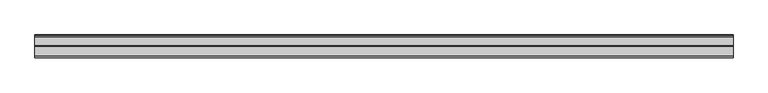
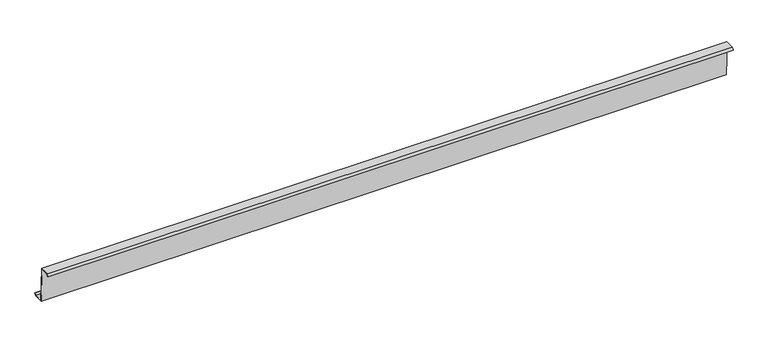
"""IFC4 building model written with IfcOpenShell, lengths in millimetres: proxy geometry, Generic Models 7:Generic Models 1:8:Generic Models 1:8 : Generic Models 7:Generic Models 1:337419:32 : Generic Models 7:Generic Models 1:8:Generic Models 1:8 : Generic Models 7:Generic Models 1:337419:315935."""

from ifc_helpers import new_model, si_unit, frame, origin, place, context, project, spatial, polyline, outline, extrude, source, transform, mapped, element, save


def generic_models_b363cb20(model_context):
    return source(origin(), model_context, "Body", "SweptSolid", [
        extrude(outline(polyline([(-574595.2827823, 4107.9663588), (-574530.4499739, 4110.6677258), (-574519.9914704, 3859.6636418), (-574459.2287164, 3862.1954233), (-574448.3924197, 3876.2595027), (-574446.191756, 3874.5639032), (-574457.8187237, 3859.4736374), (-574522.6515321, 3856.7722704), (-574533.1100356, 4107.7763544), (-574593.8424733, 4105.2458362), (-574604.690674, 4091.166307), (-574606.90975, 4092.876093), (-574595.2827823, 4107.9663588)])), frame((591306.0367239, 0.0, 0.0), z_axis=(1.0, 0.0, 0.0), x_axis=(0.0, 1.0, 0.0)), (0.0, 0.0, 1.0), 4876.8),
    ])


if __name__ == "__main__":
    model = new_model("IFC4")
    model_context = context("Model", 3, world=origin())
    ifc_project = project(units=[si_unit("LENGTHUNIT", "METRE", prefix="MILLI")], contexts=[model_context])
    site = spatial("IfcSite", under=ifc_project)
    building = spatial("IfcBuilding", under=site)
    placement = place(None, origin())
    generic_models_shape = generic_models_b363cb20(model_context)
    element("IfcBuildingElementProxy", 1, Name="Generic Models 7:Generic Models 1:8:Generic Models 1:8 : Generic Models 7:Generic Models 1:337419:32 : Generic Models 7:Generic Models 1:8:Generic Models 1:8 : Generic Models 7:Generic Models 1:337419:315935", ObjectType="Generic Models 7:Generic Models 1:8:Generic Models 1:8 : Generic Models 7:Generic Models 1:337419:32 : Generic Models 7:Generic Models 1:8:Generic Models 1:8 : Generic Models 7:Generic Models 1:337419:315935", at=placement, inside=building, context=model_context, shape_type="MappedRepresentation", body=[
        mapped(generic_models_shape, transform((0.0, 0.0, 0.0), x_axis=(1.0, 0.0, 0.0), y_axis=(0.0, 1.0, 0.0), z_axis=(0.0, 0.0, 1.0))),
    ])
    save(model, "model.ifc")

# Revit data of these elements
# Type "Generic Models 7:Generic Models 1:8:Generic Models 1:8 : Generic Models 7:Generic Models 1:337419:32 : Generic Models 7:Generic Models 1:8:Generic Models 1:8 : Generic Models 7:Generic Models 1:337419:315935"
#   NameOverride = "Generic Models 7:Generic Models 1:8:Generic Models 1:8 : Generic Models 7:Generic Models 1:337419:315935"
#   ObjectTypeOverride = "Generic Models 1:8 : Generic Models 7:Generic Models 1:337419"
#   Reference = "Generic Models 1"
#   Tag = "315935"
# Element 1 (IfcBuildingElementProxy, "Generic Models 7:Generic Models 1:8:Generic Models 1:8 : Generic Models 7:Generic Models 1:337419:32 : Generic Models 7:Generic Models 1:8:Generic Models 1:8 : Generic Models 7:Generic Models 1:337419:315935")
#   Materials on its faces: "ZEE' PURLIN (SEE STRUCT. DWGS)"
# Materials
#   "ZEE' PURLIN (SEE STRUCT. DWGS)": class "Unassigned", colour RGB 210 209 208, transparency 0, Cost = 0
